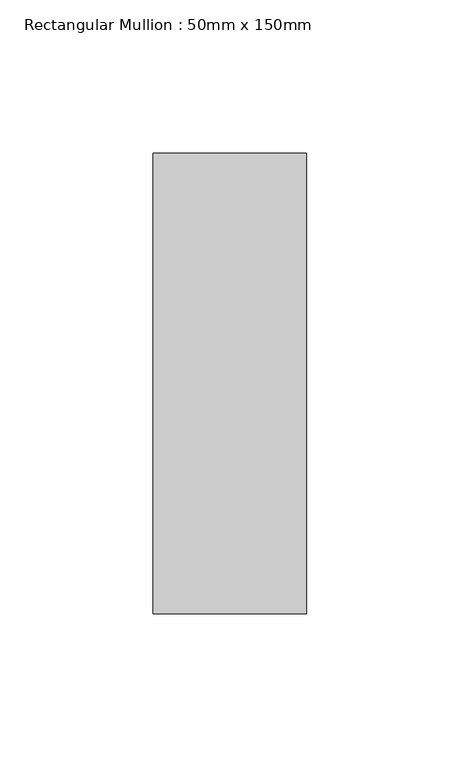
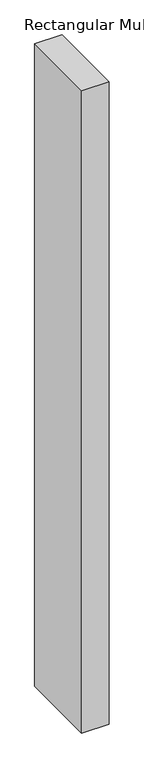
"""IFC4 building model written with IfcOpenShell, lengths in millimetres: member geometry, Rectangular Mullion : 50mm x 150mm."""

from ifc_helpers import new_model, si_unit, frame, origin, place, context, project, spatial, polyline, outline, extrude, source, transform, mapped, element, save


def rectangular_mullion_50mm_x_150mm_729c0cfc(model_context):
    return source(origin(), model_context, "Body", "SweptSolid", [
        extrude(outline(polyline([(0.0, 75.0), (0.0, -75.0), (-50.0, -75.0), (-50.0, 75.0), (0.0, 75.0)])), frame((0.0, 0.0, -1250.0), z_axis=(0.0, 0.0, 1.0), x_axis=(1.0, 0.0, 0.0)), (0.0, 0.0, 1.0), 1250.0),
    ])


if __name__ == "__main__":
    model = new_model("IFC4")
    model_context = context("Model", 3, world=origin())
    ifc_project = project(units=[si_unit("LENGTHUNIT", "METRE", prefix="MILLI")], contexts=[model_context])
    site = spatial("IfcSite", under=ifc_project)
    building = spatial("IfcBuilding", under=site)
    placement = place(None, origin())
    rectangular_mullion_50mm_x_150mm_shape = rectangular_mullion_50mm_x_150mm_729c0cfc(model_context)
    element("IfcMember", 1, ObjectType="Rectangular Mullion : 50mm x 150mm", at=placement, inside=building, context=model_context, shape_type="MappedRepresentation", body=[
        mapped(rectangular_mullion_50mm_x_150mm_shape, transform((0.0, 0.0, 0.0), x_axis=(1.0, 0.0, 0.0), y_axis=(0.0, 1.0, 0.0), z_axis=(0.0, 0.0, 1.0))),
    ])
    save(model, "model.ifc")

# Revit data of these elements
# Type "Rectangular Mullion : 50mm x 150mm"
#   built-in parameter 1007304 = 0.492126 (stored number, unit not read)
#   built-in parameter 1007301 = 0.082021 (stored number, unit not read)
#   built-in parameter 1007300 = 0.082021 (stored number, unit not read)
# Element 1 (IfcMember, "Rectangular Mullion : 50mm x 150mm")
#   Materials on its faces: "Aluminum"
# Materials
#   "Aluminum": class "Metal", colour RGB 244 244 244, transparency 0, Description = "Aluminum 6061", Cost = 0
